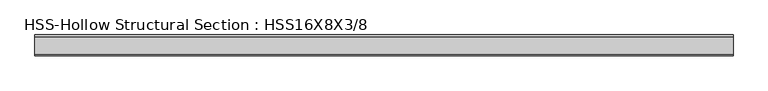
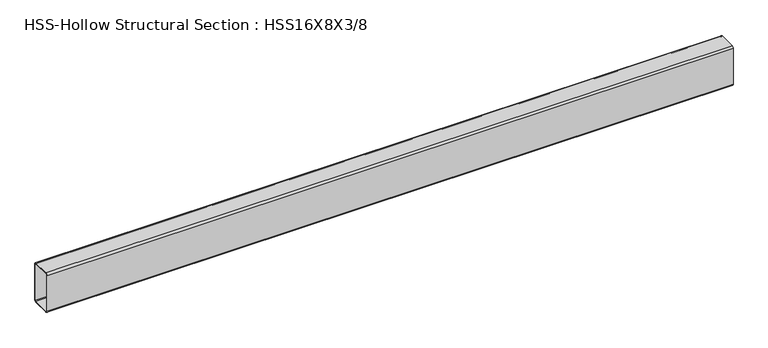
"""IFC4 building model written with IfcOpenShell, lengths in millimetres: beam geometry, HSS-Hollow Structural Section : HSS16X8X3/8."""

from ifc_helpers import new_model, si_unit, point, frame, frame_2d, origin, place, context, project, spatial, polyline, circle_curve, trimmed, segment, composite_curve, outline, extrude, source, transform, mapped, element, save


def hss_hollow_structural_section_hss16x8x3_8_50a71b2a(model_context):
    return source(origin(), model_context, "Body", "SweptSolid", [
        extrude(outline(composite_curve([segment(polyline([(101.6, 185.4708), (101.6, -185.4708)]), True, "CONTINUOUS"), segment(trimmed(circle_curve(frame_2d((83.8708, -185.4708)), 17.7292), [point((101.6, -185.4708))], [point((83.8708, -203.2))], False, "CARTESIAN"), True, "CONTINUOUS"), segment(polyline([(83.8708, -203.2), (-83.8708, -203.2)]), True, "CONTINUOUS"), segment(trimmed(circle_curve(frame_2d((-83.8708, -185.4708)), 17.7292), [point((-83.8708, -203.2))], [point((-101.6, -185.4708))], False, "CARTESIAN"), True, "CONTINUOUS"), segment(polyline([(-101.6, -185.4708), (-101.6, 185.4708)]), True, "CONTINUOUS"), segment(trimmed(circle_curve(frame_2d((-83.8708, 185.4708)), 17.7292), [point((-101.6, 185.4708))], [point((-83.8708, 203.2))], False, "CARTESIAN"), True, "CONTINUOUS"), segment(polyline([(-83.8708, 203.2), (83.8708, 203.2)]), True, "CONTINUOUS"), segment(trimmed(circle_curve(frame_2d((83.8708, 185.4708)), 17.7292), [point((83.8708, 203.2))], [point((101.6, 185.4708))], False, "CARTESIAN"), True, "CONTINUOUS")], self_intersect=False), holes=[composite_curve([segment(trimmed(circle_curve(frame_2d((-83.8708, 185.4708)), 8.8646), [point((-83.8708, 194.3354))], [point((-92.7354, 185.4708))], True, "CARTESIAN"), True, "CONTINUOUS"), segment(polyline([(-92.7354, 185.4708), (-92.7354, -185.4708)]), True, "CONTINUOUS"), segment(trimmed(circle_curve(frame_2d((-83.8708, -185.4708)), 8.8646), [point((-92.7354, -185.4708))], [point((-83.8708, -194.3354))], True, "CARTESIAN"), True, "CONTINUOUS"), segment(polyline([(-83.8708, -194.3354), (83.8708, -194.3354)]), True, "CONTINUOUS"), segment(trimmed(circle_curve(frame_2d((83.8708, -185.4708)), 8.8646), [point((83.8708, -194.3354))], [point((92.7354, -185.4708))], True, "CARTESIAN"), True, "CONTINUOUS"), segment(polyline([(92.7354, -185.4708), (92.7354, 185.4708)]), True, "CONTINUOUS"), segment(trimmed(circle_curve(frame_2d((83.8708, 185.4708)), 8.8646), [point((92.7354, 185.4708))], [point((83.8708, 194.3354))], True, "CARTESIAN"), True, "CONTINUOUS"), segment(polyline([(83.8708, 194.3354), (-83.8708, 194.3354)]), True, "CONTINUOUS")], self_intersect=False)]), frame((-3390.773, 0.0, 0.0), z_axis=(1.0, 0.0, 0.0), x_axis=(0.0, 1.0, 0.0)), (0.0, 0.0, 1.0), 6759.702),
    ])


if __name__ == "__main__":
    model = new_model("IFC4")
    model_context = context("Model", 3, world=origin())
    ifc_project = project(units=[si_unit("LENGTHUNIT", "METRE", prefix="MILLI")], contexts=[model_context])
    site = spatial("IfcSite", under=ifc_project)
    building = spatial("IfcBuilding", under=site)
    placement = place(None, origin())
    hss_hollow_structural_section_hss16x8x3_8_shape = hss_hollow_structural_section_hss16x8x3_8_50a71b2a(model_context)
    element("IfcBeam", 1, ObjectType="HSS-Hollow Structural Section : HSS16X8X3/8", at=placement, inside=building, context=model_context, shape_type="MappedRepresentation", body=[
        mapped(hss_hollow_structural_section_hss16x8x3_8_shape, transform((0.0, 0.0, 0.0), x_axis=(1.0, 0.0, 0.0), y_axis=(0.0, 1.0, 0.0), z_axis=(0.0, 0.0, 1.0))),
    ])
    save(model, "model.ifc")

# Revit data of these elements
# Type "HSS-Hollow Structural Section : HSS16X8X3/8"
#   Assembly Code = "B10"
#   Shape = "Rect."
#   W = 58.1
#   Ht = 1' - 4"
#   Length [instance default] = 5' - 0"
#   b = 0' - 8"
#   kr = 0' - 0.698"
#   t = 0' - 0.349"
#   A = 0.111111 SF
#   Structural Material [instance default] = Steel ASTM A500, Grade B, Rectangular and Square
# Element 1 (IfcBeam, "HSS-Hollow Structural Section : HSS16X8X3/8")
#   Materials on its faces: "Steel ASTM A500, Grade B, Rectangular and Square"
# Materials
#   "Steel ASTM A500, Grade B, Rectangular and Square": class "Metal", colour RGB 199 199 199, transparency 0, Description = "Carbon steel", Cost = 0
